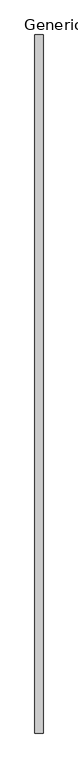
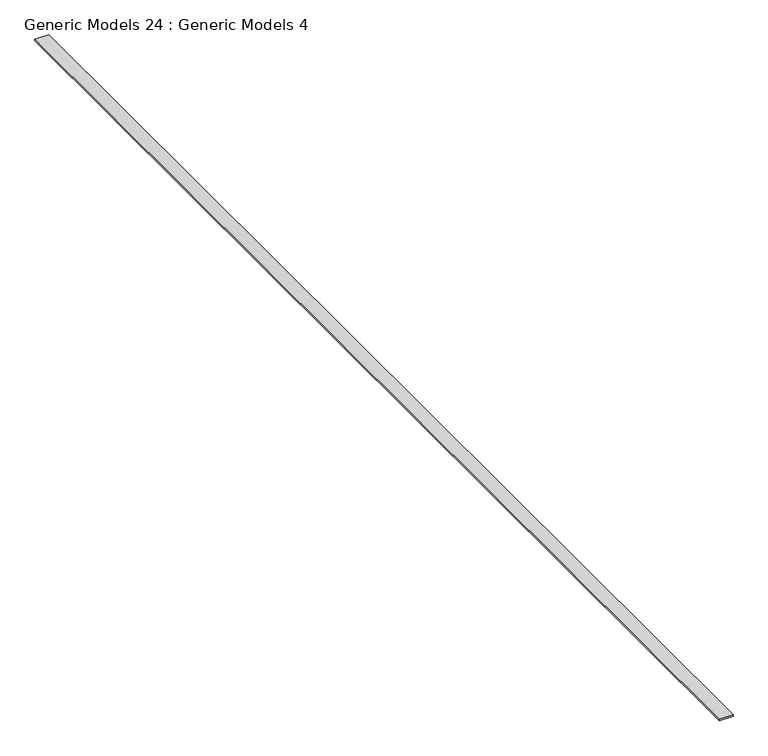
"""IFC4 building model written with IfcOpenShell, lengths in millimetres: proxy geometry, Generic Models 24 : Generic Models 4."""

from ifc_helpers import new_model, si_unit, frame, origin, place, context, project, spatial, polyline, outline, extrude, source, transform, mapped, element, save


def generic_models_24_generic_models_4_3a2b971f(model_context):
    return source(origin(), model_context, "Body", "SweptSolid", [
        extrude(outline(polyline([(8502.2047358, -2819.4174728), (8333.0059537, -2819.4174728), (8333.0059537, 11778.6769662), (8502.2047358, 11778.6769662), (8502.2047358, -2819.4174728)])), frame((0.0, 0.0, 126524.8520404), z_axis=(0.0, 0.0, 1.0), x_axis=(1.0, 0.0, 0.0)), (0.0, 0.0, 1.0), 19.05),
    ])


if __name__ == "__main__":
    model = new_model("IFC4")
    model_context = context("Model", 3, world=origin())
    ifc_project = project(units=[si_unit("LENGTHUNIT", "METRE", prefix="MILLI")], contexts=[model_context])
    site = spatial("IfcSite", under=ifc_project)
    building = spatial("IfcBuilding", under=site)
    placement = place(None, origin())
    generic_models_24_generic_models_4_shape = generic_models_24_generic_models_4_3a2b971f(model_context)
    element("IfcBuildingElementProxy", 1, Name="Generic Models 24 : Generic Models 4", ObjectType="Generic Models 24 : Generic Models 4", at=placement, inside=building, context=model_context, shape_type="MappedRepresentation", body=[
        mapped(generic_models_24_generic_models_4_shape, transform((0.0, 0.0, 0.0), x_axis=(1.0, 0.0, 0.0), y_axis=(0.0, 1.0, 0.0), z_axis=(0.0, 0.0, 1.0))),
    ])
    save(model, "model.ifc")

# Revit data of these elements
# Element 1 (IfcBuildingElementProxy, "Generic Models 24 : Generic Models 4")
#   Materials on its faces: "_CDX PLYWOOD - SEE STRUCT DWGs"
# Materials
#   "_CDX PLYWOOD - SEE STRUCT DWGs": class "Generic", colour RGB 98 75 74, transparency 0, Cost = 0
